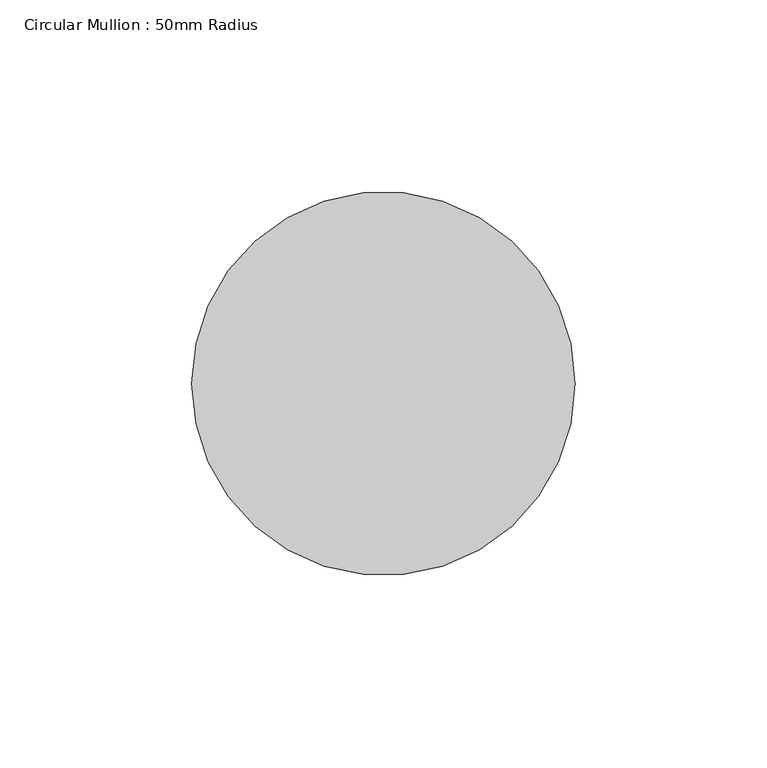
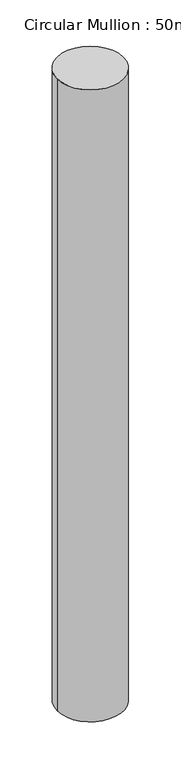
"""IFC4 building model written with IfcOpenShell, lengths in millimetres: member geometry, Circular Mullion : 50mm Radius."""

from ifc_helpers import new_model, si_unit, point, frame, origin, origin_2d, place, context, project, spatial, circle_curve, trimmed, segment, composite_curve, outline, extrude, source, transform, mapped, element, save


def circular_mullion_50mm_radius_b28a9b28(model_context):
    return source(origin(), model_context, "Body", "SweptSolid", [
        extrude(outline(composite_curve([segment(trimmed(circle_curve(origin_2d(), 50.0), [point((50.0, 0.0))], [point((-50.0, 0.0))], False, "CARTESIAN"), True, "CONTINUOUS"), segment(trimmed(circle_curve(origin_2d(), 50.0), [point((-50.0, 0.0))], [point((50.0, 0.0))], False, "CARTESIAN"), True, "CONTINUOUS")], self_intersect=False)), frame((0.0, 0.0, -1010.7789721), z_axis=(0.0, 0.0, 1.0), x_axis=(1.0, 0.0, 0.0)), (0.0, 0.0, 1.0), 1010.7789721),
    ])


if __name__ == "__main__":
    model = new_model("IFC4")
    model_context = context("Model", 3, world=origin())
    ifc_project = project(units=[si_unit("LENGTHUNIT", "METRE", prefix="MILLI")], contexts=[model_context])
    site = spatial("IfcSite", under=ifc_project)
    building = spatial("IfcBuilding", under=site)
    placement = place(None, origin())
    circular_mullion_50mm_radius_shape = circular_mullion_50mm_radius_b28a9b28(model_context)
    element("IfcMember", 1, ObjectType="Circular Mullion : 50mm Radius", at=placement, inside=building, context=model_context, shape_type="MappedRepresentation", body=[
        mapped(circular_mullion_50mm_radius_shape, transform((0.0, 0.0, 0.0), x_axis=(1.0, 0.0, 0.0), y_axis=(0.0, 1.0, 0.0), z_axis=(0.0, 0.0, 1.0))),
    ])
    save(model, "model.ifc")

# Revit data of these elements
# Type "Circular Mullion : 50mm Radius"
#   built-in parameter 1007350 = 0.164042 (stored number, unit not read)
# Element 1 (IfcMember, "Circular Mullion : 50mm Radius")
#   Materials on its faces: "Aluminium"
# Materials
#   "Aluminium": class "Metal", colour RGB 247 247 247, transparency 0, Description = "Aluminium 6061", Cost = 0
